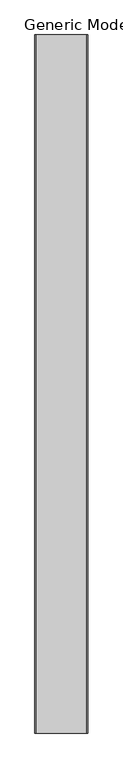
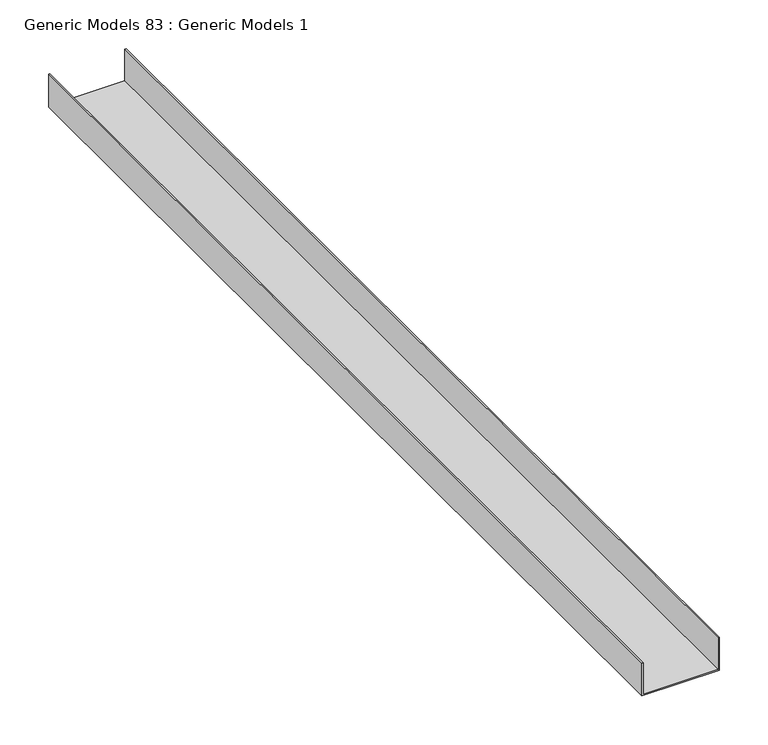
"""IFC4 building model written with IfcOpenShell, lengths in millimetres: proxy geometry, Generic Models 83 : Generic Models 1."""

from ifc_helpers import new_model, si_unit, frame, origin, place, context, project, spatial, polyline, outline, extrude, source, transform, mapped, element, save


def generic_models_83_generic_models_1_5e0949b3(model_context):
    return source(origin(), model_context, "Body", "SweptSolid", [
        extrude(outline(polyline([(142.8058091, 49802.3181639), (184.0808091, 49802.3181639), (184.0808091, 49800.7306639), (144.3933091, 49800.7306639), (144.3933091, 49711.8306639), (184.0808091, 49711.8306639), (184.0808091, 49710.2431639), (142.8058091, 49710.2431639), (142.8058091, 49802.3181639)])), frame((0.0, 0.0, 0.0), z_axis=(0.0, 1.0, 0.0), x_axis=(0.0, 0.0, 1.0)), (0.0, 0.0, 1.0), 1219.2),
    ])


if __name__ == "__main__":
    model = new_model("IFC4")
    model_context = context("Model", 3, world=origin())
    ifc_project = project(units=[si_unit("LENGTHUNIT", "METRE", prefix="MILLI")], contexts=[model_context])
    site = spatial("IfcSite", under=ifc_project)
    building = spatial("IfcBuilding", under=site)
    placement = place(None, origin())
    generic_models_83_generic_models_1_shape = generic_models_83_generic_models_1_5e0949b3(model_context)
    element("IfcBuildingElementProxy", 1, Name="Generic Models 83 : Generic Models 1", ObjectType="Generic Models 83 : Generic Models 1", at=placement, inside=building, context=model_context, shape_type="MappedRepresentation", body=[
        mapped(generic_models_83_generic_models_1_shape, transform((0.0, 0.0, 0.0), x_axis=(1.0, 0.0, 0.0), y_axis=(0.0, 1.0, 0.0), z_axis=(0.0, 0.0, 1.0))),
    ])
    save(model, "model.ifc")

# Revit data of these elements
# Element 1 (IfcBuildingElementProxy, "Generic Models 83 : Generic Models 1")
#   Materials on its faces: "DEEP LEG OF DEFLECTION TRACK (2\" MIN. DEFLECTION)"
# Materials
#   "DEEP LEG OF DEFLECTION TRACK (2\" MIN. DEFLECTION)": class "Unassigned", colour RGB 210 209 208, transparency 0, Keynote = "M05121300.02", Cost = 0
